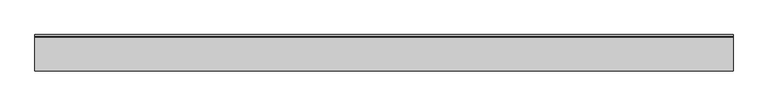
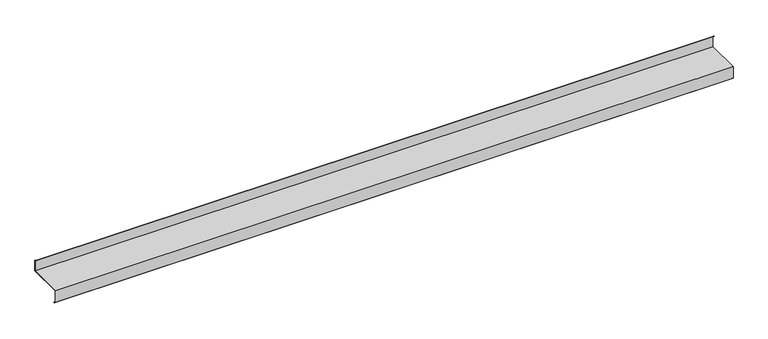
"""IFC4 building model written with IfcOpenShell, lengths in millimetres: proxy geometry, Generic Models 7:Generic Models 1:337419:Generic Models 1:337419 : Generic Models 7:Generic Models 1:337419:26 : Generic Models 7:Generic Models 1:337419:Generic Models 1:337419 : Generic Models 7:Generic Models 1:337419:301336."""

from ifc_helpers import new_model, si_unit, frame, origin, place, context, project, spatial, polyline, outline, extrude, source, transform, mapped, element, save


def generic_models_64e8c91f(model_context):
    return source(origin(), model_context, "Body", "SweptSolid", [
        extrude(outline(polyline([(-536811.2913358, 2544.5640625), (-536560.0694608, 2544.5640625), (-536560.0694608, 2619.8653956), (-536573.8564173, 2631.4340257), (-536571.8844825, 2633.4059605), (-536557.2913358, 2621.1608565), (-536557.2913358, 2541.7859375), (-536808.5132108, 2541.7859375), (-536808.5132108, 2460.1344425), (-536794.9124449, 2448.7220448), (-536796.8843797, 2446.7501099), (-536811.2913358, 2458.8389815), (-536811.2913358, 2544.5640625)])), frame((591306.0367242, 0.0, 0.0), z_axis=(1.0, 0.0, 0.0), x_axis=(0.0, 1.0, 0.0)), (0.0, 0.0, 1.0), 4876.8),
    ])


if __name__ == "__main__":
    model = new_model("IFC4")
    model_context = context("Model", 3, world=origin())
    ifc_project = project(units=[si_unit("LENGTHUNIT", "METRE", prefix="MILLI")], contexts=[model_context])
    site = spatial("IfcSite", under=ifc_project)
    building = spatial("IfcBuilding", under=site)
    placement = place(None, origin())
    generic_models_shape = generic_models_64e8c91f(model_context)
    element("IfcBuildingElementProxy", 1, Name="Generic Models 7:Generic Models 1:337419:Generic Models 1:337419 : Generic Models 7:Generic Models 1:337419:26 : Generic Models 7:Generic Models 1:337419:Generic Models 1:337419 : Generic Models 7:Generic Models 1:337419:301336", ObjectType="Generic Models 7:Generic Models 1:337419:Generic Models 1:337419 : Generic Models 7:Generic Models 1:337419:26 : Generic Models 7:Generic Models 1:337419:Generic Models 1:337419 : Generic Models 7:Generic Models 1:337419:301336", at=placement, inside=building, context=model_context, shape_type="MappedRepresentation", body=[
        mapped(generic_models_shape, transform((0.0, 0.0, 0.0), x_axis=(1.0, 0.0, 0.0), y_axis=(0.0, 1.0, 0.0), z_axis=(0.0, 0.0, 1.0))),
    ])
    save(model, "model.ifc")

# Revit data of these elements
# Type "Generic Models 7:Generic Models 1:337419:Generic Models 1:337419 : Generic Models 7:Generic Models 1:337419:26 : Generic Models 7:Generic Models 1:337419:Generic Models 1:337419 : Generic Models 7:Generic Models 1:337419:301336"
#   NameOverride = "Generic Models 7:Generic Models 1:337419:Generic Models 1:337419 : Generic Models 7:Generic Models 1:337419:301336"
#   ObjectTypeOverride = "Generic Models 1:337419 : Generic Models 7:Generic Models 1:337419"
#   Reference = "Generic Models 1"
#   Tag = "301336"
# Element 1 (IfcBuildingElementProxy, "Generic Models 7:Generic Models 1:337419:Generic Models 1:337419 : Generic Models 7:Generic Models 1:337419:26 : Generic Models 7:Generic Models 1:337419:Generic Models 1:337419 : Generic Models 7:Generic Models 1:337419:301336")
#   Materials on its faces: "'ZEE' SECTION (8.0x3.5Z - SEE STRUCT. DWGS)"
# Materials
#   "'ZEE' SECTION (8.0x3.5Z - SEE STRUCT. DWGS)": class "Unassigned", colour RGB 210 209 208, transparency 0, Keynote = "M05121300.02", Cost = 0
